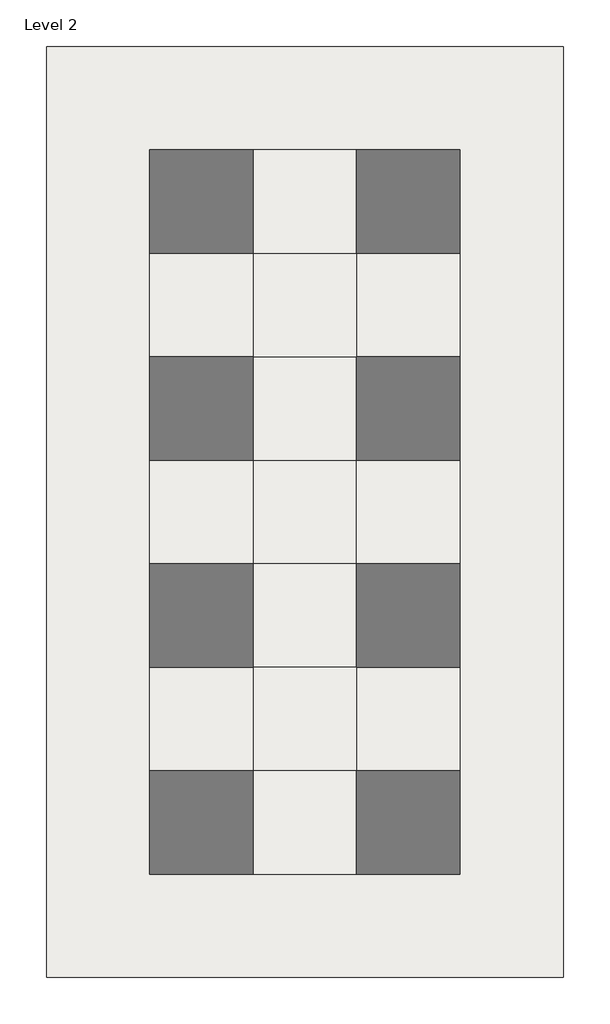
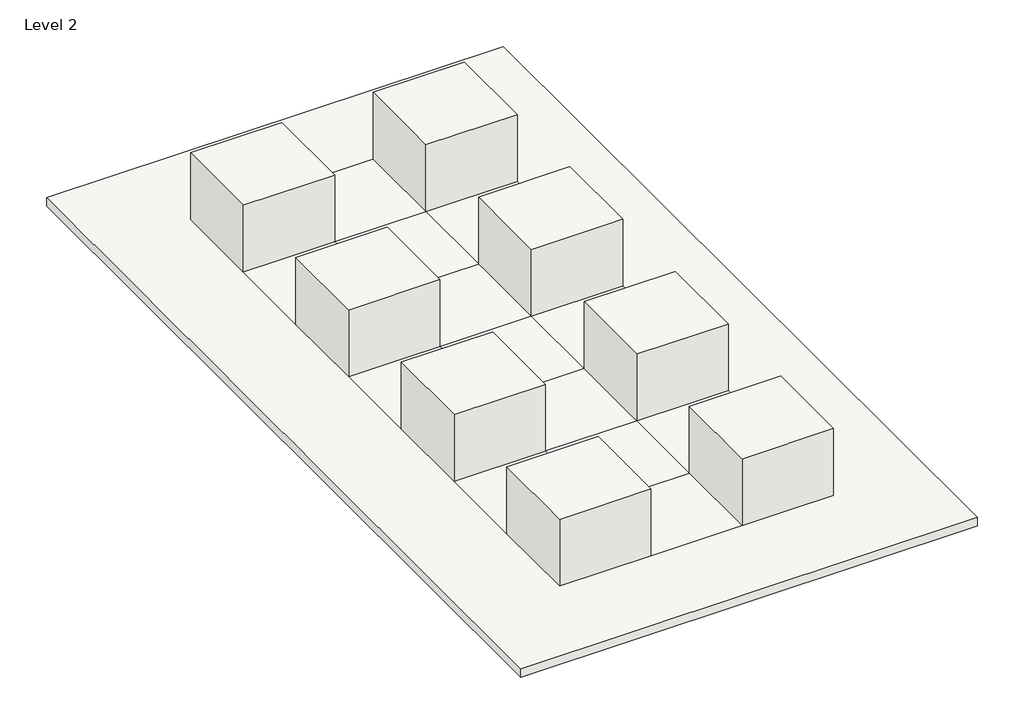
# One storey: 9 roofs.
"""IFC4 building model written with IfcOpenShell, lengths in millimetres."""

from ifc_helpers import new_model, si_unit, origin, place, context, project, spatial, faceted_brep, element, save

model = new_model("IFC4")

# Units and contexts
model_context = context("Model", 3, world=origin())
ifc_project = project(units=[si_unit("LENGTHUNIT", "METRE", prefix="MILLI")], contexts=[model_context])

# Site, building, storey
site = spatial("IfcSite", under=ifc_project)
building = spatial("IfcBuilding", under=site)
storey = spatial("IfcBuildingStorey", under=building, Name="Level 2", Elevation=8000.0)

# Roofs
placement = place(None, origin())
element("IfcRoof", 1, ObjectType="Bauder_RoofCoveringSystem_IntensiveGreenRoofSystem", at=placement, inside=storey, context=model_context, shape_type="Brep", body=[
    faceted_brep([(-674.7340554, 1676.2074539, 8000.0), (1325.2659446, 1676.2074539, 8000.0), (1325.2659446, -323.7925461, 8000.0), (-674.7340554, -323.7925461, 8000.0), (1325.2659446, 1676.2074539, 9749.8), (-674.7340554, 1676.2074539, 9749.8), (-674.7340554, -323.7925461, 9749.8), (1325.2659446, -323.7925461, 9749.8), (1325.2659446, 1676.2074539, 8200.0), (-674.7340554, 1676.2074539, 8200.0), (-674.7340554, -323.7925461, 8200.0), (1325.2659446, -323.7925461, 8200.0)], [[[0, 1, 2, 3]], [[4, 5, 6, 7]], [[5, 4, 8, 1, 0, 9]], [[6, 5, 9, 0, 3, 10]], [[7, 6, 10, 3, 2, 11]], [[4, 7, 11, 2, 1, 8]]]),
])
element("IfcRoof", 2, ObjectType="Bauder_RoofCoveringSystem_IntensiveGreenRoofSystem", at=placement, inside=storey, context=model_context, shape_type="Brep", body=[
    faceted_brep([(3325.2659446, 1676.2074539, 8000.0), (5325.2659446, 1676.2074539, 8000.0), (5325.2659446, -323.7925461, 8000.0), (3325.2659446, -323.7925461, 8000.0), (5325.2659446, 1676.2074539, 9749.8), (3325.2659446, 1676.2074539, 9749.8), (3325.2659446, -323.7925461, 9749.8), (5325.2659446, -323.7925461, 9749.8), (5325.2659446, 1676.2074539, 8200.0), (3325.2659446, 1676.2074539, 8200.0), (3325.2659446, -323.7925461, 8200.0), (5325.2659446, -323.7925461, 8200.0)], [[[0, 1, 2, 3]], [[4, 5, 6, 7]], [[5, 4, 8, 1, 0, 9]], [[6, 5, 9, 0, 3, 10]], [[7, 6, 10, 3, 2, 11]], [[4, 7, 11, 2, 1, 8]]]),
])
element("IfcRoof", 3, ObjectType="Bauder_RoofCoveringSystem_IntensiveGreenRoofSystem", at=placement, inside=storey, context=model_context, shape_type="Brep", body=[
    faceted_brep([(3325.2659446, -2323.7925461, 8000.0), (5325.2659446, -2323.7925461, 8000.0), (5325.2659446, -4323.7925461, 8000.0), (3325.2659446, -4323.7925461, 8000.0), (5325.2659446, -2323.7925461, 9749.8), (3325.2659446, -2323.7925461, 9749.8), (3325.2659446, -4323.7925461, 9749.8), (5325.2659446, -4323.7925461, 9749.8), (5325.2659446, -2323.7925461, 8200.0), (3325.2659446, -2323.7925461, 8200.0), (3325.2659446, -4323.7925461, 8200.0), (5325.2659446, -4323.7925461, 8200.0)], [[[0, 1, 2, 3]], [[4, 5, 6, 7]], [[5, 4, 8, 1, 0, 9]], [[6, 5, 9, 0, 3, 10]], [[7, 6, 10, 3, 2, 11]], [[4, 7, 11, 2, 1, 8]]]),
])
element("IfcRoof", 4, ObjectType="Bauder_RoofCoveringSystem_IntensiveGreenRoofSystem", at=placement, inside=storey, context=model_context, shape_type="Brep", body=[
    faceted_brep([(3325.2659446, -6323.7925461, 8000.0), (5325.2659446, -6323.7925461, 8000.0), (5325.2659446, -8323.7925461, 8000.0), (3325.2659446, -8323.7925461, 8000.0), (5325.2659446, -6323.7925461, 9749.8), (3325.2659446, -6323.7925461, 9749.8), (3325.2659446, -8323.7925461, 9749.8), (5325.2659446, -8323.7925461, 9749.8), (5325.2659446, -6323.7925461, 8200.0), (3325.2659446, -6323.7925461, 8200.0), (3325.2659446, -8323.7925461, 8200.0), (5325.2659446, -8323.7925461, 8200.0)], [[[0, 1, 2, 3]], [[4, 5, 6, 7]], [[5, 4, 8, 1, 0, 9]], [[6, 5, 9, 0, 3, 10]], [[7, 6, 10, 3, 2, 11]], [[4, 7, 11, 2, 1, 8]]]),
])
element("IfcRoof", 5, ObjectType="Bauder_RoofCoveringSystem_IntensiveGreenRoofSystem", at=placement, inside=storey, context=model_context, shape_type="Brep", body=[
    faceted_brep([(3325.2659446, -10323.7925461, 8000.0), (5325.2659446, -10323.7925461, 8000.0), (5325.2659446, -12323.7925461, 8000.0), (3325.2659446, -12323.7925461, 8000.0), (5325.2659446, -10323.7925461, 9749.8), (3325.2659446, -10323.7925461, 9749.8), (3325.2659446, -12323.7925461, 9749.8), (5325.2659446, -12323.7925461, 9749.8), (5325.2659446, -10323.7925461, 8200.0), (3325.2659446, -10323.7925461, 8200.0), (3325.2659446, -12323.7925461, 8200.0), (5325.2659446, -12323.7925461, 8200.0)], [[[0, 1, 2, 3]], [[4, 5, 6, 7]], [[5, 4, 8, 1, 0, 9]], [[6, 5, 9, 0, 3, 10]], [[7, 6, 10, 3, 2, 11]], [[4, 7, 11, 2, 1, 8]]]),
])
element("IfcRoof", 6, ObjectType="Bauder_RoofCoveringSystem_IntensiveGreenRoofSystem", at=placement, inside=storey, context=model_context, shape_type="Brep", body=[
    faceted_brep([(-674.7340554, -10323.7925461, 8000.0), (1325.2659446, -10323.7925461, 8000.0), (1325.2659446, -12323.7925461, 8000.0), (-674.7340554, -12323.7925461, 8000.0), (1325.2659446, -10323.7925461, 9749.8), (-674.7340554, -10323.7925461, 9749.8), (-674.7340554, -12323.7925461, 9749.8), (1325.2659446, -12323.7925461, 9749.8), (1325.2659446, -10323.7925461, 8200.0), (-674.7340554, -10323.7925461, 8200.0), (-674.7340554, -12323.7925461, 8200.0), (1325.2659446, -12323.7925461, 8200.0)], [[[0, 1, 2, 3]], [[4, 5, 6, 7]], [[5, 4, 8, 1, 0, 9]], [[6, 5, 9, 0, 3, 10]], [[7, 6, 10, 3, 2, 11]], [[4, 7, 11, 2, 1, 8]]]),
])
element("IfcRoof", 7, ObjectType="Bauder_RoofCoveringSystem_IntensiveGreenRoofSystem", at=placement, inside=storey, context=model_context, shape_type="Brep", body=[
    faceted_brep([(-674.7340554, -6323.7925461, 8000.0), (1325.2659446, -6323.7925461, 8000.0), (1325.2659446, -8323.7925461, 8000.0), (-674.7340554, -8323.7925461, 8000.0), (1325.2659446, -6323.7925461, 9749.8), (-674.7340554, -6323.7925461, 9749.8), (-674.7340554, -8323.7925461, 9749.8), (1325.2659446, -8323.7925461, 9749.8), (1325.2659446, -6323.7925461, 8200.0), (-674.7340554, -6323.7925461, 8200.0), (-674.7340554, -8323.7925461, 8200.0), (1325.2659446, -8323.7925461, 8200.0)], [[[0, 1, 2, 3]], [[4, 5, 6, 7]], [[5, 4, 8, 1, 0, 9]], [[6, 5, 9, 0, 3, 10]], [[7, 6, 10, 3, 2, 11]], [[4, 7, 11, 2, 1, 8]]]),
])
element("IfcRoof", 8, ObjectType="Bauder_RoofCoveringSystem_IntensiveGreenRoofSystem", at=placement, inside=storey, context=model_context, shape_type="Brep", body=[
    faceted_brep([(-674.7340554, -2323.7925461, 8000.0), (1325.2659446, -2323.7925461, 8000.0), (1325.2659446, -4323.7925461, 8000.0), (-674.7340554, -4323.7925461, 8000.0), (1325.2659446, -2323.7925461, 9749.8), (-674.7340554, -2323.7925461, 9749.8), (-674.7340554, -4323.7925461, 9749.8), (1325.2659446, -4323.7925461, 9749.8), (1325.2659446, -2323.7925461, 8200.0), (-674.7340554, -2323.7925461, 8200.0), (-674.7340554, -4323.7925461, 8200.0), (1325.2659446, -4323.7925461, 8200.0)], [[[0, 1, 2, 3]], [[4, 5, 6, 7]], [[5, 4, 8, 1, 0, 9]], [[6, 5, 9, 0, 3, 10]], [[7, 6, 10, 3, 2, 11]], [[4, 7, 11, 2, 1, 8]]]),
])
element("IfcRoof", 9, ObjectType="Roof_Concrete-200mm", at=placement, inside=storey, context=model_context, shape_type="Brep", body=[
    faceted_brep([(-2674.7340554, -14323.7925461, 8200.0), (-2674.7340554, -14323.7925461, 8000.0), (7325.2659446, -14323.7925461, 8000.0), (7325.2659446, -14323.7925461, 8200.0), (-2674.7340554, 3676.2074539, 8200.0), (-2674.7340554, 3676.2074539, 8000.0), (7325.2659446, 3676.2074539, 8200.0), (7325.2659446, 3676.2074539, 8000.0), (3325.2659446, 1676.2074539, 8200.0), (1325.2659446, 1676.2074539, 8200.0), (1325.2659446, -323.7925461, 8200.0), (3325.2659446, -323.7925461, 8200.0), (1325.2659446, 1676.2074539, 8000.0), (3325.2659446, 1676.2074539, 8000.0), (3325.2659446, -323.7925461, 8000.0), (1325.2659446, -323.7925461, 8000.0), (1325.2659446, -2323.7925461, 8200.0), (-674.7340554, -323.7925461, 8200.0), (-674.7340554, -2323.7925461, 8200.0), (3325.2659446, -2323.7925461, 8200.0), (5325.2659446, -2323.7925461, 8200.0), (5325.2659446, -323.7925461, 8200.0), (-674.7340554, -2323.7925461, 8000.0), (-674.7340554, -323.7925461, 8000.0), (1325.2659446, -2323.7925461, 8000.0), (3325.2659446, -2323.7925461, 8000.0), (5325.2659446, -323.7925461, 8000.0), (5325.2659446, -2323.7925461, 8000.0), (1325.2659446, -4323.7925461, 8200.0), (3325.2659446, -4323.7925461, 8200.0), (3325.2659446, -4323.7925461, 8000.0), (1325.2659446, -4323.7925461, 8000.0), (1325.2659446, -6323.7925461, 8200.0), (-674.7340554, -4323.7925461, 8200.0), (-674.7340554, -6323.7925461, 8200.0), (5325.2659446, -6323.7925461, 8200.0), (5325.2659446, -4323.7925461, 8200.0), (3325.2659446, -6323.7925461, 8200.0), (-674.7340554, -6323.7925461, 8000.0), (-674.7340554, -4323.7925461, 8000.0), (1325.2659446, -6323.7925461, 8000.0), (3325.2659446, -6323.7925461, 8000.0), (5325.2659446, -4323.7925461, 8000.0), (5325.2659446, -6323.7925461, 8000.0), (1325.2659446, -12323.7925461, 8200.0), (3325.2659446, -12323.7925461, 8200.0), (3325.2659446, -10323.7925461, 8200.0), (1325.2659446, -10323.7925461, 8200.0), (3325.2659446, -12323.7925461, 8000.0), (1325.2659446, -12323.7925461, 8000.0), (1325.2659446, -10323.7925461, 8000.0), (3325.2659446, -10323.7925461, 8000.0), (1325.2659446, -8323.7925461, 8200.0), (-674.7340554, -8323.7925461, 8200.0), (-674.7340554, -10323.7925461, 8200.0), (3325.2659446, -8323.7925461, 8200.0), (5325.2659446, -10323.7925461, 8200.0), (5325.2659446, -8323.7925461, 8200.0), (-674.7340554, -10323.7925461, 8000.0), (-674.7340554, -8323.7925461, 8000.0), (1325.2659446, -8323.7925461, 8000.0), (3325.2659446, -8323.7925461, 8000.0), (5325.2659446, -8323.7925461, 8000.0), (5325.2659446, -10323.7925461, 8000.0), (-674.7340554, 1676.2074539, 8000.0), (-674.7340554, 1676.2074539, 8200.0), (5325.2659446, 1676.2074539, 8200.0), (5325.2659446, 1676.2074539, 8000.0), (5325.2659446, -12323.7925461, 8000.0), (5325.2659446, -12323.7925461, 8200.0), (-674.7340554, -12323.7925461, 8000.0), (-674.7340554, -12323.7925461, 8200.0)], [[[0, 1, 2, 3]], [[1, 0, 4, 5]], [[6, 7, 5, 4]], [[3, 2, 7, 6]], [[8, 9, 10, 11]], [[12, 13, 14, 15]], [[16, 10, 17, 18]], [[11, 10, 16, 19]], [[20, 21, 11, 19]], [[22, 23, 15, 24]], [[15, 14, 25, 24]], [[25, 14, 26, 27]], [[19, 16, 28, 29]], [[24, 25, 30, 31]], [[32, 28, 33, 34]], [[35, 36, 29, 37]], [[38, 39, 31, 40]], [[41, 30, 42, 43]], [[44, 45, 46, 47]], [[48, 49, 50, 51]], [[47, 52, 53, 54]], [[47, 46, 55, 52]], [[56, 57, 55, 46]], [[58, 59, 60, 50]], [[51, 50, 60, 61]], [[51, 61, 62, 63]], [[52, 55, 37, 32]], [[29, 28, 32, 37]], [[61, 60, 40, 41]], [[31, 30, 41, 40]], [[9, 12, 15, 10]], [[10, 15, 23, 17]], [[17, 23, 64, 65]], [[12, 9, 65, 64]], [[66, 67, 26, 21]], [[21, 26, 14, 11]], [[11, 14, 13, 8]], [[67, 66, 8, 13]], [[20, 27, 42, 36]], [[36, 42, 30, 29]], [[29, 30, 25, 19]], [[27, 20, 19, 25]], [[16, 24, 31, 28]], [[28, 31, 39, 33]], [[33, 39, 22, 18]], [[24, 16, 18, 22]], [[32, 40, 60, 52]], [[52, 60, 59, 53]], [[53, 59, 38, 34]], [[40, 32, 34, 38]], [[35, 43, 62, 57]], [[57, 62, 61, 55]], [[55, 61, 41, 37]], [[43, 35, 37, 41]], [[56, 63, 68, 69]], [[69, 68, 48, 45]], [[45, 48, 51, 46]], [[63, 56, 46, 51]], [[47, 50, 49, 44]], [[44, 49, 70, 71]], [[71, 70, 58, 54]], [[50, 47, 54, 58]], [[4, 0, 3, 6], [9, 8, 66, 21, 20, 36, 35, 57, 56, 69, 45, 44, 71, 54, 53, 34, 33, 18, 17, 65]], [[7, 2, 1, 5], [13, 12, 64, 23, 22, 39, 38, 59, 58, 70, 49, 48, 68, 63, 62, 43, 42, 27, 26, 67]]]),
])

save(model, "model.ifc")

# Revit data of these elements
# Type "Bauder_RoofCoveringSystem_IntensiveGreenRoofSystem"
#   Keynote = "Q37"
#   Type IFC Predefined Type = "FLAT_ROOF"
#   Export Type to IFC As = "IfcRoofType"
#   Model = "Bauder Intensive Landscaping and Substrate - Intensive Green Roof System"
#   Manufacturer = "Bauder Ltd"
#   Type Comments = "Intensive Green Roof System"
#   URL = "http://www.bauder.co.uk/"
#   Description = "Bauder Intensive GreenRoof system incorporating Intensive Landscaping with Intensive Substrate, Filter Fleece, Mineral Drain, DSE60 Polyethylene Drainage and Protection Layer, FSM 1100 protection mat and PE Foil Polyethylene Separation-Slip Layer"
#   Assembly Code = "B3010"
#   NBSDescription = "Intensive green roof system"
#   NBSReference = "45-40-47/110"
#   BIMObjectName = "Bauder_RoofCoveringSystem_IntensiveGreenRoofSystem"
#   AccessibilityPerformance = "n/a"
#   CodePerformance = "n/a"
#   Color = "n/a"
#   Constituents = "n/a"
#   DurationUnit = "Year"
#   ExpectedLife = "n/a"
#   Features = "This BIM Object must be supported by a project specific specification from Bauder, incorporating system build-up, detail design and performance calculations if a full Bauder system guarantee is required. Please contact your local Bauder Representative or technical@bauder.co.uk"
#   Finish = "n/a"
#   Grade = "n/a"
#   Material = "n/a"
#   ModelReference = "Bauder Intensive Landscaping and Substrate - Intensive Green Roof System"
#   Name = "RoofCoveringSystem_Bauder_IntensiveGreenRoofSystem"
#   ReplacementCost = "n/a"
#   Shape = "n/a"
#   Size = "n/a"
#   SustainabilityPerformance = "Bauder Germany ISO14001: Certificate No.: 70499/03-15 e, Bauder UK ISO14001:Certificate No. 19ACM6595R, EN1271, BREEAM Credits Available"
#   WarrantyDescription = "Guarantee options could include ‘Product’, ‘Product and Workmanship’ and ‘Product, Workmanship and Design’ Guarantees. All guarantees available for this system are subject to the works being carried out in accordance with the Bauder specification and being installed by a Bauder Approved installer. For full details and further information regarding guarantees and alternative systems please contact your local Bauder Representative or technical@bauder.co.uk"
#   WarrantyDurationLabor = "n/a"
#   WarrantyDurationParts = "n/a\r\nn/a"
#   WarrantyDurationUnit = "Year"
#   WarrantyGuarantorLabor = "n/a"
#   WarrantyGuarantorParts = "technical@bauder.co.uk"
#   Certification = "n/a"
#   EdgeRestraints = "Perforated edge trim where required, refer to Bauder Project Specific Specification"
#   MoistureControlDrainageAncillaries = "n/a"
#   MoistureControlDrainageLayer = "Bauder DSE60 60 mm Polyethylene Drainage and Protection Layer with Bauder Mineral Drain Single size stone aggregate infill"
#   MoistureControlFilterMembrane = "Bauder Filter Fleece 1 mm Polypropylene Filter Fleece"
#   MoistureControlMoistureRetentionMat = "n/a"
#   PlantingSystemsAntierosionMat = "Jute Net where exposed, refer to Bauder Project Specific Specification"
#   PlantingSystemsPlantingMedium = "Bauder Intensive Substrate Recycled crushed brick, expanded clay shale and composted pine bark"
#   PlantingSystemsVegetation = "Bauder Intensive Landscaping"
#   PlantingSystemsVegetationBarrier = "20-40 mm Rounded-Washed Stones, refer to Bauder Project Specific Specification"
#   ProjectSpecificationAndDesign = "This BIM Object must be supported by a project specific specification from Bauder, incorporating system build-up, detail design and performance calculations if a full Bauder system warranty is required. Please contact your local Bauder Representative or technical@bauder.co.uk"
#   ProtectionProtectionLayer = "BauderGREEN FSM 1100 Protection Mat"
#   ProtectionRootBarrier = "As per project specific Bauder Specification"
#   ProtectionSeparationLayer = "2 layers of Bauder PE Foil 0.2 mm Polyethylene Separation-Slip Layer"
#   SystemManufacturer = "Bauder Ltd"
#   WarrantyConsiderations = "All guarantees available for this system are subject to the works being carried out in accordance with the Bauder specification and being installed by a Bauder Approved installer. For full details and further information regarding guarantees and alternative systems please contact your local Bauder Representative or technical@bauder.co.uk"
#   Update = "1900-12-31T23:59:59"
#   Documentation = "https://www.bauder.co.uk/technical-centre/technical-literature/system-brochures"
#   DocumentReference = "http://www.bauder.co.uk/"
#   IfcExportAs = "IfcRoofType"
#   IfcExportType = "FLAT_ROOF"
#   MethodOfMesurement = "n/a"
#   Process = "Replacement at service life intervals"
#   FireRating = "n/a"
#   _Author = "AM"
#   _AuthorizedBy = "bimstore"
#   _CreatedBy = "technical@bauder.co.uk"
#   _DistributedBy = "www.bimstore.co"
#   AssetType = "Fixed"
#   ClassificationName = "Uniclass2015"
#   ClassificationValue = "Ss_45_40_47_40"
#   CreatedBy = "technical@bauder.co.uk"
#   CreatedOn = "2023-02-10 T00:00:00"
#   DocumentationCertificates = "n/a"
#   DocumentationInstallationGuide = "https://www.bauder.co.uk/technical-centre"
#   DocumentationLiterature = "https://www.bauder.co.uk/technical-centre"
#   DocumentationMaintenance = "https://www.bauder.co.uk/technical-centre/maintenance-advice"
#   DocumentationTechnical = "https://www.bauder.co.uk/green-roofs/intensive-green-roofs"
#   ManufacturerName = "Bauder Ltd"
#   ModelNumber = "0910_INT-InS-FF-D6-F11-PE"
#   ProductionYear = "2023"
#   ReferencedStandard = "n/a"
#   SpareParts = "n/a"
#   TypeName = "Intensive Green Roof System"
#   NBSNote = "n/a"
#   NBSObjectName = "Bauder - Intensive green roof system"
#   NBSOfficeMasterTag = "n/a"
#   Ballast = "n/a"
#   CarrierMembraneFixing = "n/a"
#   CarrierMembraneType = "n/a"
#   FillToPerimeterUpstands = "n/a"
#   FilterLayer = "n/a"
#   InsulationFixing = "n/a"
#   InsulationType = "n/a"
#   LiquidAppliedWaterproofCoatingReinforcement = "n/a"
#   LiquidAppliedWaterproofCoatingSurfaceTreatment = "n/a"
#   LiquidAppliedWaterproofCoatingType = "n/a"
#   PreparationExistingSubstrates = "n/a"
#   PreparationHorizontalWork = "n/a"
#   PreparationSkirtingsAndVerticalWork = "n/a"
#   ProtectionLayer = "n/a"
#   SystemAccessories = "n/a"
#   WaterproofCoveringFirstLayerAttachment = "n/a"
#   WaterproofCoveringFirstLayerType = "n/a"
#   WaterproofCoveringIntermediateLayerAttachment = "n/a"
#   WaterproofCoveringIntermediateLayerType = "n/a"
#   WaterproofCoveringTopLayerAttachment = "n/a"
#   InsulationAttachment = "n/a"
#   IsolatingLayer = "n/a"
#   CarrierMembraneAttachment = "n/a"
#   LiquidAppliedWaterproofCoatingWearingCourse = "n/a"
#   VapourControlLayer = "n/a"
#   VapourControlLayerAttachment_Bauder = "n/a"
#   WaterproofCoveringJoints = "n/a"
#   WaterproofCoveringType = "n/a"
#   SeparatingLayer = "n/a"
#   WaterproofCoveringAccessories = "Yes"
#   WaterproofCoveringAttachment = "n/a"
#   UpperProtectionLayer = "n/a"
#   LowerProtectionLayer = "n/a"
#   WaterproofCoveringTopLayerType = "n/a"
#   DetailWorkAncillaryItems = "Detail as per project specific Bauder Specification"
#   DetailWorkCoverStrips = "Detail as per project specific Bauder Specification"
#   DetailWorkFlashings = "Detail as per project specific Bauder Specification"
#   DetailWorkSkirtingsAndUpstands = "Detail as per project specific Bauder Specification"
#   DetailWorkWeltedDrips = "Detail as per project specific Bauder Specification"
#   OverlayFixing = "n/a"
#   OverlayType = "n/a"
#   SurfaceProtection = "n/a"
#   VapourControlLayerAttachment = "n/a"
#   VapourControlLayerType = "n/a"
#   Cost = 0
#   NominalHeight = 0 mm
#   NominalLength = 0 mm
#   TotalArea = 0 m²
#   NominalDepth = 0 mm
#   IsExternal = yes
#   _BimSpecGuid = 0
#   _BSBibleVersion = 16
#   _CurrentRevision = 4
#   Layers, outside or top first: 700 mm "Bauder_Landscaping_Intensive" (function 5); 800 mm "Bauder_IntensiveSubstrate_BauderGREEN-SUB-IM-UK" (function 2); 1 mm "Bauder_FilterFleece_BauderGREEN-FV-125-100" (function 2); 40 mm "Bauder_DrainageBoard_BauderGREEN-DSE-40" (function 3); 8 mm "Bauder_ProtectionMat_BauderGREEN-FSM1100" (function 3); 200 mm "Concrete" (function 1); 0.8 mm "Bauder_SeparationAndSlipLayer_BauderGREEN-PE-02" (function 3)
# Type "Roof_Concrete-200mm"
#   Layers, outside or top first: 200 mm "Concrete" (function 1)
# Elements 1, 2, 3, 4, 5, 6, 7, 8 (IfcRoof, "Bauder_RoofCoveringSystem_IntensiveGreenRoofSystem")
#   built-in parameter 1001705 = 31.9875 (stored number, unit not read)
#   built-in parameter 1001710 = 33615
#   Phase Created = New Construction
#   Materials on its faces: "Bauder_SeparationAndSlipLayer_BauderGREEN-PE-02", "Bauder_Landscaping_Intensive"
# Element 9 (IfcRoof, "Roof_Concrete-200mm")
#   built-in parameter 1001710 = 33615
#   Phase Created = New Construction
#   Materials on its faces: "Concrete"
# Materials
#   "Bauder_Landscaping_Intensive": class "Unassigned", colour RGB 62 68 37, transparency 0, Mtrl_Author = "AM", Mtrl_AuthorizedBy = "bimstore", Mtrl_DistributedBy = "www.bimstore.co", Mtrl_AccessibilityPerformance = "n/a", Mtrl_AssetIdentifier = "Please record on commissioning", Mtrl_AssetType = "Fixed", Mtrl_BarCode = "Please record on commissioning", Mtrl_ClassificationName = "Uniclass2015", Mtrl_ClassificationValue = "n/a", Mtrl_CodePerformance = "n/a", Mtrl_Color = "n/a", Mtrl_Constituents = "n/a", Mtrl_CreatedBy = "technical@bauder.co.uk", Mtrl_CreatedOn = "2023-02-10 T00:00:00", Mtrl_DocumentationCertificates = "https://www.bimstore.co/products/intensive-green-roof-system/document/product-certificates", Mtrl_DocumentationInstallationGuide = "https://www.bimstore.co/products/intensive-green-roof-system/document/installation-guide", Mtrl_DocumentationLiterature = "https://www.bimstore.co/products/intensive-green-roof-system/document/product-literature", Mtrl_DocumentationMaintenance = "https://www.bimstore.co/products/intensive-green-roof-system/document/maintenance-information", Mtrl_DocumentationTechnical = "https://www.bimstore.co/products/intensive-green-roof-system/document/technical-data-sheet", Mtrl_DurationUnit = "Year", Mtrl_Features = "n/a", Mtrl_Finish = "n/a", Mtrl_Grade = "n/a", Mtrl_InstallationDate = "Please record on commissioning", Mtrl_ManufacturerName = "Bauder Ltd", Mtrl_Material = "n/a", Mtrl_ModelNumber = "Intensive", Mtrl_ModelReference = "Landscaping", Mtrl_ProductionYear = "2023", Mtrl_ReferencedStandard = "n/a", Mtrl_Shape = "n/a", Mtrl_Size = "n/a", Mtrl_SpareParts = "n/a", Mtrl_TypeName = "Intensive", Mtrl_WarrantyDescription = "n/a", Mtrl_WarrantyDurationUnit = "Year", Mtrl_WarrantyGuarantorLabor = "n/a", Mtrl_WarrantyGuarantorParts = "technical@bauder.co.uk", Mtrl_WarrantyStartDate = "Please record on commissioning", Mtrl_IfcExportAs = "IfcRoofType", Mtrl_IfcExportType = "FLAT_ROOF", Mtrl_BIMObjectName = "Bauder_Landscaping_Intensive", Mtrl_NBSDescription = "n/a", Mtrl_NBSNote = "n/a", Mtrl_NBSObjectName = "n/a", Mtrl_NBSOfficeMasterTag = "n/a", Mtrl_NBSReference = "Q37", Mtrl_Ballast = "n/a", Mtrl_CarrierMembraneAttachment = "n/a", Mtrl_CarrierMembraneFixing = "n/a", Mtrl_CarrierMembraneType = "n/a", Mtrl_Certification = "Comply with GRO Green Roof Code of Practice and FLL Standards", Mtrl_DetailWorkAncillaryItems = "Detail as per project specific Bauder Specification", Mtrl_DetailWorkCoverStrips = "Detail as per project specific Bauder Specification", Mtrl_DetailWorkFlashings = "Detail as per project specific Bauder Specification", Mtrl_DetailWorkSkirtingsAndUpstands = "Detail as per project specific Bauder Specification", Mtrl_DetailWorkWeltedDrips = "Detail as per project specific Bauder Specification", Mtrl_EdgeRestraints = "Detail as per project specific Bauder Specification", Mtrl_FillToPerimeterUpstands = "n/a", Mtrl_FilterLayer = "n/a", Mtrl_InsulationAttachment = "As per project specific Bauder Specification", Mtrl_InsulationFixing = "As per project specific Bauder Specification", Mtrl_InsulationType = "As per project specific Bauder Specification", Mtrl_IsolatingLayer = "n/a", Mtrl_LiquidAppliedWaterproofCoatingReinforcement = "n/a", Mtrl_LiquidAppliedWaterproofCoatingSurfaceTreatment = "As per project specific Bauder Specification", Mtrl_LiquidAppliedWaterproofCoatingType = "As per project specific Bauder Specification", Mtrl_LiquidAppliedWaterproofCoatingWearingCourse = "As per project specific Bauder Specification", Mtrl_LowerProtectionLayer = "n/a", Mtrl_MoistureControlDrainageAncillaries = "n/a", Mtrl_MoistureControlDrainageLayer = "n/a", Mtrl_MoistureControlFilterMembrane = "n/a", Mtrl_MoistureControlMoistureRetentionMat = "n/a", Mtrl_OverlayFixing = "n/a", Mtrl_OverlayType = "n/a", Mtrl_PlantingSystemsAntierosionMat = "n/a", Mtrl_PlantingSystemsPlantingMedium = "As per project specific Bauder Specification", Mtrl_PlantingSystemsVegetation = "As per project specific Bauder Specification", Mtrl_PlantingSystemsVegetationBarrier = "As per project specific Bauder Specification", Mtrl_PreparationExistingSubstrates = "n/a", Mtrl_PreparationHorizontalWork = "n/a", Mtrl_PreparationSkirtingsAndVerticalWork = "n/a", Mtrl_ProjectSpecificationAndDesign = "This BIM Object must be supported by a project specific specification from Bauder, incorporating system build-up, detail design and performance calculations if a full Bauder system warranty is required. Please contact your local Bauder Representative or technical@bauder.co.uk", Mtrl_ProtectionLayer = "n/a", Mtrl_ProtectionProtectionLayer = "n/a", Mtrl_ProtectionRootBarrier = "As per project specific Bauder Specification", Mtrl_ProtectionSeparationLayer = "n/a", Mtrl_SeparatingLayer = "n/a", Mtrl_SurfaceProtection = "n/a", Mtrl_SystemAccessories = "n/a", Mtrl_SystemManufacturer = "Bauder Ltd", Mtrl_Update = "1900-12-31 T23:59:59", Mtrl_UpperProtectionLayer = "n/a", Mtrl_VapourControlLayerAttachment = "As per project specific Bauder Specification", Mtrl_VapourControlLayerAttachment_Bauder = "As per project specific Bauder Specification", Mtrl_VapourControlLayerType = "As per project specific Bauder Specification", Mtrl_WarrantyConsiderations = "All guarantees available for this system are subject to the works being carried out in accordance with the Bauder specification and being installed by a Bauder Approved installer. For full details and further information regarding guarantees and alternative systems please contact your local Bauder Representative or technical@bauder.co.uk", Mtrl_WaterproofCoveringAccessories = "As per project specific Bauder Specification", Mtrl_WaterproofCoveringAttachment = "As per project specific Bauder Specification", Mtrl_WaterproofCoveringFirstLayerAttachment = "As per project specific Bauder Specification", Mtrl_WaterproofCoveringFirstLayerType = "As per project specific Bauder Specification", Mtrl_WaterproofCoveringIntermediateLayerAttachment = "As per project specific Bauder Specification", Mtrl_WaterproofCoveringIntermediateLayerType = "As per project specific Bauder Specification", Mtrl_WaterproofCoveringJoints = "As per project specific Bauder Specification", Mtrl_WaterproofCoveringTopLayerAttachment = "As per project specific Bauder Specification", Mtrl_WaterproofCoveringTopLayerType = "As per project specific Bauder Specification", Mtrl_WaterproofCoveringType = "As per project specific Bauder Specification", Cost = 0, Mtrl_ReplacementCost = 0, Mtrl_NominalDepth = 0 mm, Mtrl_NominalHeight = 0 mm, Mtrl_NominalLength = 0 mm, Mtrl_BimSpecGuid = 0, Mtrl_BSBibleVersion = 17, Mtrl_CurrentRevision = 2, Mtrl_ExpectedLife = 0, Mtrl_SerialNumber = 0, Mtrl_WarrantyDurationLabor = 0, Mtrl_WarrantyDurationParts = 0
#   "Bauder_IntensiveSubstrate_BauderGREEN-SUB-IM-UK": class "Unassigned", colour RGB 255 255 255, transparency 0, Mtrl_Author = "AM", Mtrl_AuthorizedBy = "bimstore", Mtrl_DistributedBy = "www.bimstore.co", Mtrl_AccessibilityPerformance = "n/a", Mtrl_AssetIdentifier = "Please record on commissioning", Mtrl_AssetType = "Fixed", Mtrl_BarCode = "Please record on commissioning", Mtrl_ClassificationName = "Uniclass2015", Mtrl_ClassificationValue = "n/a", Mtrl_CodePerformance = "n/a", Mtrl_Color = "n/a", Mtrl_Constituents = "n/a", Mtrl_CreatedBy = "technical@bauder.co.uk", Mtrl_CreatedOn = "2023-02-10 T00:00:00", Mtrl_DocumentationCertificates = "https://www.bimstore.co/products/intensive-green-roof-system/document/product-certificates", Mtrl_DocumentationInstallationGuide = "https://www.bimstore.co/products/intensive-green-roof-system/document/installation-guide", Mtrl_DocumentationLiterature = "https://www.bimstore.co/products/intensive-green-roof-system/document/product-literature", Mtrl_DocumentationMaintenance = "https://www.bimstore.co/products/intensive-green-roof-system/document/maintenance-information", Mtrl_DocumentationTechnical = "https://www.bimstore.co/products/intensive-green-roof-system/document/technical-data-sheet", Mtrl_DurationUnit = "Year", Mtrl_Features = "n/a", Mtrl_Finish = "n/a", Mtrl_Grade = "n/a", Mtrl_InstallationDate = "Please record on commissioning", Mtrl_ManufacturerName = "Bauder Ltd", Mtrl_Material = "Expanded Clay Aggregate", Mtrl_ModelNumber = "BauderGREEN-SUB-IM-UK", Mtrl_ModelReference = "Intensive Substrate", Mtrl_ProductionYear = "2023", Mtrl_ReferencedStandard = "n/a", Mtrl_Shape = "n/a", Mtrl_Size = "n/a", Mtrl_SpareParts = "n/a", Mtrl_TypeName = "BauderGREEN-SUB-IM-UK", Mtrl_WarrantyDescription = "As part of Bauder system guarantee, per specification", Mtrl_WarrantyDurationUnit = "Year", Mtrl_WarrantyGuarantorLabor = "n/a", Mtrl_WarrantyGuarantorParts = "technical@bauder.co.uk", Mtrl_WarrantyStartDate = "Please record on commissioning", Mtrl_IfcExportAs = "IfcRoofType", Mtrl_IfcExportType = "FLAT_ROOF", Mtrl_BIMObjectName = "Bauder_IntensiveSubstrate_BauderGREEN-SUB-IM-UK", Mtrl_NBSDescription = "n/a", Mtrl_NBSNote = "n/a", Mtrl_NBSObjectName = "n/a", Mtrl_NBSOfficeMasterTag = "n/a", Mtrl_NBSReference = "Q37", Mtrl_Ballast = "n/a", Mtrl_CarrierMembraneAttachment = "n/a", Mtrl_CarrierMembraneFixing = "n/a", Mtrl_CarrierMembraneType = "n/a", Mtrl_Certification = "Comply with GRO Green Roof Code of Practice and FLL Standards", Mtrl_DetailWorkAncillaryItems = "Detail as per project specific Bauder Specification", Mtrl_DetailWorkCoverStrips = "Detail as per project specific Bauder Specification", Mtrl_DetailWorkFlashings = "Detail as per project specific Bauder Specification", Mtrl_DetailWorkSkirtingsAndUpstands = "Detail as per project specific Bauder Specification", Mtrl_DetailWorkWeltedDrips = "Detail as per project specific Bauder Specification", Mtrl_EdgeRestraints = "Detail as per project specific Bauder Specification", Mtrl_FillToPerimeterUpstands = "n/a", Mtrl_FilterLayer = "n/a", Mtrl_InsulationAttachment = "As per project specific Bauder Specification", Mtrl_InsulationFixing = "As per project specific Bauder Specification", Mtrl_InsulationType = "As per project specific Bauder Specification", Mtrl_IsolatingLayer = "n/a", Mtrl_LiquidAppliedWaterproofCoatingReinforcement = "As per project specific Bauder Specification", Mtrl_LiquidAppliedWaterproofCoatingSurfaceTreatment = "As per project specific Bauder Specification", Mtrl_LiquidAppliedWaterproofCoatingType = "As per project specific Bauder Specification", Mtrl_LiquidAppliedWaterproofCoatingWearingCourse = "As per project specific Bauder Specification", Mtrl_LowerProtectionLayer = "n/a", Mtrl_MoistureControlDrainageAncillaries = "n/a", Mtrl_MoistureControlDrainageLayer = "n/a", Mtrl_MoistureControlFilterMembrane = "n/a", Mtrl_MoistureControlMoistureRetentionMat = "n/a", Mtrl_OverlayFixing = "n/a", Mtrl_OverlayType = "n/a", Mtrl_PlantingSystemsAntierosionMat = "n/a", Mtrl_PlantingSystemsPlantingMedium = "As per project specific Bauder Specification", Mtrl_PlantingSystemsVegetation = "As per project specific Bauder Specification", Mtrl_PlantingSystemsVegetationBarrier = "As per project specific Bauder Specification", Mtrl_PreparationExistingSubstrates = "n/a", Mtrl_PreparationHorizontalWork = "n/a", Mtrl_PreparationSkirtingsAndVerticalWork = "n/a", Mtrl_ProjectSpecificationAndDesign = "This BIM Object must be supported by a project specific specification from Bauder, incorporating system build-up, detail design and performance calculations if a full Bauder system warranty is required. Please contact your local Bauder Representative or technical@bauder.co.uk", Mtrl_ProtectionLayer = "n/a", Mtrl_ProtectionProtectionLayer = "n/a", Mtrl_ProtectionRootBarrier = "As per project specific Bauder Specification", Mtrl_ProtectionSeparationLayer = "n/a", Mtrl_SeparatingLayer = "n/a", Mtrl_SurfaceProtection = "n/a", Mtrl_SystemAccessories = "n/a", Mtrl_SystemManufacturer = "Bauder Ltd", Mtrl_Update = "1900-12-31 T23:59:59", Mtrl_UpperProtectionLayer = "n/a", Mtrl_VapourControlLayerAttachment = "As per project specific Bauder Specification", Mtrl_VapourControlLayerAttachment_Bauder = "As per project specific Bauder Specification", Mtrl_VapourControlLayerType = "As per project specific Bauder Specification", Mtrl_WarrantyConsiderations = "All guarantees available for this system are subject to the works being carried out in accordance with the Bauder specification and being installed by a Bauder Approved installer. For full details and further information regarding guarantees and alternative systems please contact your local Bauder Representative or technical@bauder.co.uk", Mtrl_WaterproofCoveringAccessories = "As per project specific Bauder Specification", Mtrl_WaterproofCoveringAttachment = "As per project specific Bauder Specification", Mtrl_WaterproofCoveringFirstLayerAttachment = "As per project specific Bauder Specification", Mtrl_WaterproofCoveringFirstLayerType = "As per project specific Bauder Specification", Mtrl_WaterproofCoveringIntermediateLayerAttachment = "As per project specific Bauder Specification", Mtrl_WaterproofCoveringIntermediateLayerType = "As per project specific Bauder Specification", Mtrl_WaterproofCoveringJoints = "As per project specific Bauder Specification", Mtrl_WaterproofCoveringTopLayerAttachment = "As per project specific Bauder Specification", Mtrl_WaterproofCoveringTopLayerType = "As per project specific Bauder Specification", Mtrl_WaterproofCoveringType = "As per project specific Bauder Specification", Cost = 0, Mtrl_ReplacementCost = 0, Mtrl_NominalDepth = 200 mm, Mtrl_NominalHeight = 0 mm, Mtrl_NominalLength = 0 mm, Mtrl_BimSpecGuid = 0, Mtrl_BSBibleVersion = 17, Mtrl_CurrentRevision = 2, Mtrl_ExpectedLife = 0, Mtrl_SerialNumber = 0, Mtrl_WarrantyDurationLabor = 0, Mtrl_WarrantyDurationParts = 0
#   "Bauder_FilterFleece_BauderGREEN-FV-125-100": class "Unassigned", colour RGB 255 255 255, transparency 0, Mtrl_Author = "AM", Mtrl_AuthorizedBy = "bimstore", Mtrl_DistributedBy = "www.bimstore.co", Mtrl_AccessibilityPerformance = "n/a", Mtrl_AssetIdentifier = "Please record on commissioning", Mtrl_AssetType = "Fixed", Mtrl_BarCode = "Please record on commissioning", Mtrl_ClassificationName = "Uniclass2015", Mtrl_ClassificationValue = "n/a", Mtrl_CodePerformance = "n/a", Mtrl_Color = "n/a", Mtrl_Constituents = "n/a", Mtrl_CreatedBy = "technical@bauder.co.uk", Mtrl_CreatedOn = "2023-02-10 T00:00:00", Mtrl_DocumentationCertificates = "https://www.bimstore.co/products/extensive-green-roof-system-wildflower-blanket/document/product-certificates", Mtrl_DocumentationInstallationGuide = "https://www.bimstore.co/products/extensive-green-roof-system-wildflower-blanket/document/installation-guide", Mtrl_DocumentationLiterature = "https://www.bimstore.co/products/intensive-green-roof-system/document/product-literature", Mtrl_DocumentationMaintenance = "https://www.bimstore.co/products/extensive-green-roof-system-wildflower-blanket/document/maintenance-information", Mtrl_DocumentationTechnical = "https://www.bimstore.co/products/extensive-green-roof-system-wildflower-blanket/document/technical-data-sheet", Mtrl_DurationUnit = "Year", Mtrl_Features = "n/a", Mtrl_Finish = "n/a", Mtrl_Grade = "n/a", Mtrl_InstallationDate = "Please record on commissioning", Mtrl_ManufacturerName = "Bauder Ltd", Mtrl_Material = "Polypropylene Fleece", Mtrl_ModelNumber = "BauderGREEN-FV-125-100", Mtrl_ModelReference = "Filter Fleece", Mtrl_ProductionYear = "2023", Mtrl_ReferencedStandard = "n/a", Mtrl_Shape = "n/a", Mtrl_Size = "n/a", Mtrl_SpareParts = "n/a", Mtrl_TypeName = "BauderGREEN-FV-125-100", Mtrl_WarrantyDescription = "As part of Bauder system guarantee, per specification", Mtrl_WarrantyDurationUnit = "Year", Mtrl_WarrantyGuarantorLabor = "technical@bauder.co.uk", Mtrl_WarrantyGuarantorParts = "technical@bauder.co.uk", Mtrl_WarrantyStartDate = "Please record on commissioning", Mtrl_IfcExportAs = "IfcRoofType", Mtrl_IfcExportType = "FLAT_ROOF", Mtrl_BIMObjectName = "Bauder_FilterFleece_BauderGREEN-FV-125-100", Mtrl_NBSDescription = "n/a", Mtrl_NBSNote = "n/a", Mtrl_NBSObjectName = "n/a", Mtrl_NBSOfficeMasterTag = "n/a", Mtrl_NBSReference = "Q37", Mtrl_Ballast = "n/a", Mtrl_CarrierMembraneAttachment = "n/a", Mtrl_CarrierMembraneFixing = "n/a", Mtrl_CarrierMembraneType = "n/a", Mtrl_Certification = "Comply with GRO Green Roof Code of Practice and FLL Standards", Mtrl_DetailWorkAncillaryItems = "Detail as per project specific Bauder Specification", Mtrl_DetailWorkCoverStrips = "Detail as per project specific Bauder Specification", Mtrl_DetailWorkFlashings = "Detail as per project specific Bauder Specification", Mtrl_DetailWorkSkirtingsAndUpstands = "Detail as per project specific Bauder Specification", Mtrl_DetailWorkWeltedDrips = "Detail as per project specific Bauder Specification", Mtrl_EdgeRestraints = "Detail as per project specific Bauder Specification", Mtrl_FillToPerimeterUpstands = "n/a", Mtrl_FilterLayer = "n/a", Mtrl_InsulationAttachment = "As per project specific Bauder Specification", Mtrl_InsulationFixing = "As per project specific Bauder Specification", Mtrl_InsulationType = "As per project specific Bauder Specification", Mtrl_IsolatingLayer = "n/a", Mtrl_LiquidAppliedWaterproofCoatingReinforcement = "As per project specific Bauder Specification", Mtrl_LiquidAppliedWaterproofCoatingSurfaceTreatment = "As per project specific Bauder Specification", Mtrl_LiquidAppliedWaterproofCoatingType = "As per project specific Bauder Specification", Mtrl_LiquidAppliedWaterproofCoatingWearingCourse = "As per project specific Bauder Specification", Mtrl_LowerProtectionLayer = "n/a", Mtrl_MoistureControlDrainageAncillaries = "n/a", Mtrl_MoistureControlDrainageLayer = "n/a", Mtrl_MoistureControlFilterMembrane = "n/a", Mtrl_MoistureControlMoistureRetentionMat = "n/a", Mtrl_OverlayFixing = "n/a", Mtrl_OverlayType = "n/a", Mtrl_PlantingSystemsAntierosionMat = "n/a", Mtrl_PlantingSystemsPlantingMedium = "As per project specific Bauder Specification", Mtrl_PlantingSystemsVegetation = "As per project specific Bauder Specification", Mtrl_PlantingSystemsVegetationBarrier = "As per project specific Bauder Specification", Mtrl_PreparationExistingSubstrates = "n/a", Mtrl_PreparationHorizontalWork = "n/a", Mtrl_PreparationSkirtingsAndVerticalWork = "n/a", Mtrl_ProjectSpecificationAndDesign = "This BIM Object must be supported by a project specific specification from Bauder, incorporating system build-up, detail design and performance calculations if a full Bauder system warranty is required. Please contact your local Bauder Representative or technical@bauder.co.uk", Mtrl_ProtectionLayer = "n/a", Mtrl_ProtectionProtectionLayer = "n/a", Mtrl_ProtectionRootBarrier = "As per project specific Bauder Specification", Mtrl_ProtectionSeparationLayer = "n/a", Mtrl_SeparatingLayer = "n/a", Mtrl_SurfaceProtection = "n/a", Mtrl_SystemAccessories = "n/a", Mtrl_SystemManufacturer = "Bauder Ltd", Mtrl_Update = "1900-12-31 T23:59:59", Mtrl_UpperProtectionLayer = "n/a", Mtrl_VapourControlLayerAttachment = "As per project specific Bauder Specification", Mtrl_VapourControlLayerAttachment_Bauder = "As per project specific Bauder Specification", Mtrl_VapourControlLayerType = "As per project specific Bauder Specification", Mtrl_WarrantyConsiderations = "All guarantees available for this system are subject to the works being carried out in accordance with the Bauder specification and being installed by a Bauder Approved installer. For full details and further information regarding guarantees and alternative systems please contact your local Bauder Representative or technical@bauder.co.uk", Mtrl_WaterproofCoveringAccessories = "As per project specific Bauder Specification", Mtrl_WaterproofCoveringAttachment = "As per project specific Bauder Specification", Mtrl_WaterproofCoveringFirstLayerAttachment = "As per project specific Bauder Specification", Mtrl_WaterproofCoveringFirstLayerType = "As per project specific Bauder Specification", Mtrl_WaterproofCoveringIntermediateLayerAttachment = "As per project specific Bauder Specification", Mtrl_WaterproofCoveringIntermediateLayerType = "As per project specific Bauder Specification", Mtrl_WaterproofCoveringJoints = "As per project specific Bauder Specification", Mtrl_WaterproofCoveringTopLayerAttachment = "As per project specific Bauder Specification", Mtrl_WaterproofCoveringTopLayerType = "As per project specific Bauder Specification", Mtrl_WaterproofCoveringType = "As per project specific Bauder Specification", Cost = 0, Mtrl_ReplacementCost = 0, Mtrl_NominalDepth = 1 mm, Mtrl_NominalHeight = 0 mm, Mtrl_NominalLength = 0 mm, Mtrl_BimSpecGuid = 0, Mtrl_BSBibleVersion = 17, Mtrl_CurrentRevision = 2, Mtrl_ExpectedLife = 0, Mtrl_SerialNumber = 0, Mtrl_WarrantyDurationLabor = 0, Mtrl_WarrantyDurationParts = 0
#   "Bauder_DrainageBoard_BauderGREEN-DSE-40": class "Unassigned", colour RGB 255 255 255, transparency 0, Mtrl_Author = "AM", Mtrl_AuthorizedBy = "bimstore", Mtrl_DistributedBy = "www.bimstore.co", Mtrl_AccessibilityPerformance = "n/a", Mtrl_AssetIdentifier = "Please record on commissioning", Mtrl_AssetType = "Fixed", Mtrl_BarCode = "Please record on commissioning", Mtrl_ClassificationName = "Uniclass2015", Mtrl_ClassificationValue = "Pr_65_67_78_72", Mtrl_CodePerformance = "n/a", Mtrl_Color = "n/a", Mtrl_Constituents = "n/a", Mtrl_CreatedBy = "technical@bauder.co.uk", Mtrl_CreatedOn = "2023-02-10 T00:00:00", Mtrl_DocumentationCertificates = "https://www.bimstore.co/products/extensive-green-roof-system-wildflower-blanket/document/product-certificates", Mtrl_DocumentationInstallationGuide = "https://www.bimstore.co/products/extensive-green-roof-system-wildflower-blanket/document/installation-guide", Mtrl_DocumentationLiterature = "https://www.bimstore.co/products/extensive-green-roof-system-wildflower-blanket/document/product-literature", Mtrl_DocumentationMaintenance = "https://www.bimstore.co/products/extensive-green-roof-system-wildflower-blanket/document/maintenance-information", Mtrl_DocumentationTechnical = "https://www.bimstore.co/products/extensive-green-roof-system-wildflower-blanket/document/technical-data-sheet", Mtrl_DurationUnit = "Year", Mtrl_Features = "n/a", Mtrl_Finish = "n/a", Mtrl_Grade = "n/a", Mtrl_InstallationDate = "Please record on commissioning", Mtrl_ManufacturerName = "Bauder Ltd", Mtrl_Material = "Recycled High Density Polyethylene", Mtrl_ModelNumber = "BauderGREEN-DSE-40", Mtrl_ModelReference = "Drainage Board", Mtrl_ProductionYear = "2023", Mtrl_ReferencedStandard = "n/a", Mtrl_Shape = "n/a", Mtrl_Size = "n/a", Mtrl_SpareParts = "n/a", Mtrl_TypeName = "BauderGREEN-DSE-40", Mtrl_WarrantyDescription = "As part of Bauder system guarantee, per specification", Mtrl_WarrantyDurationUnit = "Year", Mtrl_WarrantyGuarantorLabor = "technical@bauder.co.uk", Mtrl_WarrantyGuarantorParts = "technical@bauder.co.uk", Mtrl_WarrantyStartDate = "Please record on commissioning", Mtrl_IfcExportAs = "IfcRoofType", Mtrl_IfcExportType = "FLAT_ROOF", Mtrl_BIMObjectName = "Bauder_DrainageBoard_BauderGREEN-DSE-40", Mtrl_NBSDescription = "n/a", Mtrl_NBSNote = "n/a", Mtrl_NBSObjectName = "n/a", Mtrl_NBSOfficeMasterTag = "n/a", Mtrl_NBSReference = "Q37", Mtrl_Ballast = "n/a", Mtrl_CarrierMembraneAttachment = "n/a", Mtrl_CarrierMembraneFixing = "n/a", Mtrl_CarrierMembraneType = "n/a", Mtrl_Certification = "Comply with GRO Green Roof Code of Practice and FLL Standards", Mtrl_DetailWorkAncillaryItems = "Detail as per project specific Bauder Specification", Mtrl_DetailWorkCoverStrips = "Detail as per project specific Bauder Specification", Mtrl_DetailWorkFlashings = "Detail as per project specific Bauder Specification", Mtrl_DetailWorkSkirtingsAndUpstands = "Detail as per project specific Bauder Specification", Mtrl_DetailWorkWeltedDrips = "Detail as per project specific Bauder Specification", Mtrl_EdgeRestraints = "Detail as per project specific Bauder Specification", Mtrl_FillToPerimeterUpstands = "n/a", Mtrl_FilterLayer = "n/a", Mtrl_InsulationAttachment = "As per project specific Bauder Specification", Mtrl_InsulationFixing = "As per project specific Bauder Specification", Mtrl_InsulationType = "As per project specific Bauder Specification", Mtrl_IsolatingLayer = "n/a", Mtrl_LiquidAppliedWaterproofCoatingReinforcement = "As per project specific Bauder Specification", Mtrl_LiquidAppliedWaterproofCoatingSurfaceTreatment = "As per project specific Bauder Specification", Mtrl_LiquidAppliedWaterproofCoatingType = "As per project specific Bauder Specification", Mtrl_LiquidAppliedWaterproofCoatingWearingCourse = "As per project specific Bauder Specification", Mtrl_LowerProtectionLayer = "n/a", Mtrl_MoistureControlDrainageAncillaries = "n/a", Mtrl_MoistureControlDrainageLayer = "n/a", Mtrl_MoistureControlFilterMembrane = "n/a", Mtrl_MoistureControlMoistureRetentionMat = "n/a", Mtrl_OverlayFixing = "n/a", Mtrl_OverlayType = "n/a", Mtrl_PlantingSystemsAntierosionMat = "n/a", Mtrl_PlantingSystemsPlantingMedium = "As per project specific Bauder Specification", Mtrl_PlantingSystemsVegetation = "As per project specific Bauder Specification", Mtrl_PlantingSystemsVegetationBarrier = "As per project specific Bauder Specification", Mtrl_PreparationExistingSubstrates = "n/a", Mtrl_PreparationHorizontalWork = "n/a", Mtrl_PreparationSkirtingsAndVerticalWork = "n/a", Mtrl_ProjectSpecificationAndDesign = "This BIM Object must be supported by a project specific specification from Bauder, incorporating system build-up, detail design and performance calculations if a full Bauder system warranty is required. Please contact your local Bauder Representative or technical@bauder.co.uk", Mtrl_ProtectionLayer = "n/a", Mtrl_ProtectionProtectionLayer = "n/a", Mtrl_ProtectionRootBarrier = "As per project specific Bauder Specification", Mtrl_ProtectionSeparationLayer = "n/a", Mtrl_SeparatingLayer = "n/a", Mtrl_SurfaceProtection = "n/a", Mtrl_SystemAccessories = "n/a", Mtrl_SystemManufacturer = "Bauder Ltd", Mtrl_Update = "1900-12-31 T23:59:59", Mtrl_UpperProtectionLayer = "n/a", Mtrl_VapourControlLayerAttachment = "As per project specific Bauder Specification", Mtrl_VapourControlLayerAttachment_Bauder = "As per project specific Bauder Specification", Mtrl_VapourControlLayerType = "As per project specific Bauder Specification", Mtrl_WarrantyConsiderations = "All guarantees available for this system are subject to the works being carried out in accordance with the Bauder specification and being installed by a Bauder Approved installer. For full details and further information regarding guarantees and alternative systems please contact your local Bauder Representative or technical@bauder.co.uk", Mtrl_WaterproofCoveringAccessories = "As per project specific Bauder Specification", Mtrl_WaterproofCoveringAttachment = "As per project specific Bauder Specification", Mtrl_WaterproofCoveringFirstLayerAttachment = "As per project specific Bauder Specification", Mtrl_WaterproofCoveringFirstLayerType = "As per project specific Bauder Specification", Mtrl_WaterproofCoveringIntermediateLayerAttachment = "As per project specific Bauder Specification", Mtrl_WaterproofCoveringIntermediateLayerType = "As per project specific Bauder Specification", Mtrl_WaterproofCoveringJoints = "As per project specific Bauder Specification", Mtrl_WaterproofCoveringTopLayerAttachment = "As per project specific Bauder Specification", Mtrl_WaterproofCoveringTopLayerType = "As per project specific Bauder Specification", Mtrl_WaterproofCoveringType = "As per project specific Bauder Specification", Cost = 0, Mtrl_ReplacementCost = 0, Mtrl_NominalDepth = 40 mm, Mtrl_NominalHeight = 0 mm, Mtrl_NominalLength = 0 mm, Mtrl_BimSpecGuid = 0, Mtrl_BSBibleVersion = 17, Mtrl_CurrentRevision = 2, Mtrl_ExpectedLife = 0, Mtrl_SerialNumber = 0, Mtrl_WarrantyDurationLabor = 0, Mtrl_WarrantyDurationParts = 0
#   "Bauder_ProtectionMat_BauderGREEN-FSM1100": class "Unassigned", colour RGB 255 255 255, transparency 0, Mtrl_Author = "AM", Mtrl_AuthorizedBy = "bimstore", Mtrl_DistributedBy = "www.bimstore.co", Mtrl_AccessibilityPerformance = "n/a", Mtrl_AssetIdentifier = "Please record on commissioning", Mtrl_AssetType = "Fixed", Mtrl_BarCode = "Please record on commissioning", Mtrl_ClassificationName = "Uniclass2015", Mtrl_ClassificationValue = "Pr_20_96_71_64", Mtrl_CodePerformance = "n/a", Mtrl_Color = "n/a", Mtrl_Constituents = "n/a", Mtrl_CreatedBy = "technical@bauder.co.uk", Mtrl_CreatedOn = "2023-05-02 T00:00:00", Mtrl_DocumentationCertificates = "https://www.bimstore.co/products/intensive-green-roof-system/document/product-certificates", Mtrl_DocumentationInstallationGuide = "https://www.bimstore.co/products/intensive-green-roof-system/document/installation-guide", Mtrl_DocumentationLiterature = "https://www.bimstore.co/products/intensive-green-roof-system/document/product-literature", Mtrl_DocumentationMaintenance = "https://www.bimstore.co/products/intensive-green-roof-system/document/maintenance-information", Mtrl_DocumentationTechnical = "https://www.bimstore.co/products/intensive-green-roof-system/document/technical-data-sheet", Mtrl_DurationUnit = "Year", Mtrl_Features = "n/a", Mtrl_Finish = "n/a", Mtrl_Grade = "n/a", Mtrl_InstallationDate = "Please record on commissioning", Mtrl_ManufacturerName = "Bauder Ltd", Mtrl_Material = "Polyester and Polypropylene Fibre", Mtrl_ModelNumber = "BauderGREEN FSM1100", Mtrl_ModelReference = "Protection Mat", Mtrl_ProductionYear = "2023", Mtrl_ReferencedStandard = "n/a", Mtrl_Shape = "n/a", Mtrl_Size = "n/a", Mtrl_SpareParts = "n/a", Mtrl_TypeName = "BauderGREEN FSM1100", Mtrl_WarrantyDescription = "As part of Bauder system guarantee, per specification", Mtrl_WarrantyDurationUnit = "Year", Mtrl_WarrantyGuarantorLabor = "n/a", Mtrl_WarrantyGuarantorParts = "technical@bauder.co.uk", Mtrl_WarrantyStartDate = "Please record on commissioning", Mtrl_IfcExportAs = "IfcRoofType", Mtrl_IfcExportType = "FLAT_ROOF", Mtrl_BIMObjectName = "Bauder_ProtectionMat_BauderGREEN-FSM1100", Mtrl_NBSDescription = "n/a", Mtrl_NBSNote = "n/a", Mtrl_NBSObjectName = "n/a", Mtrl_NBSOfficeMasterTag = "n/a", Mtrl_NBSReference = "Q37", Mtrl_Ballast = "n/a", Mtrl_CarrierMembraneAttachment = "n/a", Mtrl_CarrierMembraneFixing = "n/a", Mtrl_CarrierMembraneType = "n/a", Mtrl_Certification = "Comply with GRO Green Roof Code of Practice and FLL Standards", Mtrl_DetailWorkAncillaryItems = "Detail as per project specific Bauder Specification", Mtrl_DetailWorkCoverStrips = "Detail as per project specific Bauder Specification", Mtrl_DetailWorkFlashings = "Detail as per project specific Bauder Specification", Mtrl_DetailWorkSkirtingsAndUpstands = "Detail as per project specific Bauder Specification", Mtrl_DetailWorkWeltedDrips = "Detail as per project specific Bauder Specification", Mtrl_EdgeRestraints = "Detail as per project specific Bauder Specification", Mtrl_FillToPerimeterUpstands = "n/a", Mtrl_FilterLayer = "n/a", Mtrl_InsulationAttachment = "As per project specific Bauder Specification", Mtrl_InsulationFixing = "As per project specific Bauder Specification", Mtrl_InsulationType = "As per project specific Bauder Specification", Mtrl_IsolatingLayer = "n/a", Mtrl_LiquidAppliedWaterproofCoatingReinforcement = "As per project specific Bauder Specification", Mtrl_LiquidAppliedWaterproofCoatingSurfaceTreatment = "As per project specific Bauder Specification", Mtrl_LiquidAppliedWaterproofCoatingType = "As per project specific Bauder Specification", Mtrl_LiquidAppliedWaterproofCoatingWearingCourse = "As per project specific Bauder Specification", Mtrl_LowerProtectionLayer = "n/a", Mtrl_MoistureControlDrainageAncillaries = "n/a", Mtrl_MoistureControlDrainageLayer = "n/a", Mtrl_MoistureControlFilterMembrane = "n/a", Mtrl_MoistureControlMoistureRetentionMat = "n/a", Mtrl_OverlayFixing = "n/a", Mtrl_OverlayType = "n/a", Mtrl_PlantingSystemsAntierosionMat = "n/a", Mtrl_PlantingSystemsPlantingMedium = "As per project specific Bauder Specification", Mtrl_PlantingSystemsVegetation = "As per project specific Bauder Specification", Mtrl_PlantingSystemsVegetationBarrier = "As per project specific Bauder Specification", Mtrl_PreparationExistingSubstrates = "n/a", Mtrl_PreparationHorizontalWork = "n/a", Mtrl_PreparationSkirtingsAndVerticalWork = "n/a", Mtrl_ProjectSpecificationAndDesign = "This BIM Object must be supported by a project specific specification from Bauder, incorporating system build-up, detail design and performance calculations if a full Bauder system warranty is required. Please contact your local Bauder Representative or technical@bauder.co.uk", Mtrl_ProtectionLayer = "n/a", Mtrl_ProtectionProtectionLayer = "n/a", Mtrl_ProtectionRootBarrier = "As per project specific Bauder Specification", Mtrl_ProtectionSeparationLayer = "n/a", Mtrl_SeparatingLayer = "n/a", Mtrl_SurfaceProtection = "n/a", Mtrl_SystemAccessories = "n/a", Mtrl_SystemManufacturer = "Bauder Ltd", Mtrl_Update = "1900-12-31 T23:59:59", Mtrl_UpperProtectionLayer = "n/a", Mtrl_VapourControlLayerAttachment = "As per project specific Bauder Specification", Mtrl_VapourControlLayerAttachment_Bauder = "As per project specific Bauder Specification", Mtrl_VapourControlLayerType = "As per project specific Bauder Specification", Mtrl_WarrantyConsiderations = "All guarantees available for this system are subject to the works being carried out in accordance with the Bauder specification and being installed by a Bauder Approved installer. For full details and further information regarding guarantees and alternative systems please contact your local Bauder Representative or technical@bauder.co.uk", Mtrl_WaterproofCoveringAccessories = "As per project specific Bauder Specification", Mtrl_WaterproofCoveringAttachment = "As per project specific Bauder Specification", Mtrl_WaterproofCoveringFirstLayerAttachment = "As per project specific Bauder Specification", Mtrl_WaterproofCoveringFirstLayerType = "As per project specific Bauder Specification", Mtrl_WaterproofCoveringIntermediateLayerAttachment = "As per project specific Bauder Specification", Mtrl_WaterproofCoveringIntermediateLayerType = "As per project specific Bauder Specification", Mtrl_WaterproofCoveringJoints = "As per project specific Bauder Specification", Mtrl_WaterproofCoveringTopLayerAttachment = "As per project specific Bauder Specification", Mtrl_WaterproofCoveringTopLayerType = "As per project specific Bauder Specification", Mtrl_WaterproofCoveringType = "As per project specific Bauder Specification", Cost = 0, Mtrl_ReplacementCost = 0, Mtrl_NominalDepth = 8 mm, Mtrl_NominalHeight = 0 mm, Mtrl_NominalLength = 0 mm, Mtrl_BimSpecGuid = 0, Mtrl_BSBibleVersion = 17, Mtrl_CurrentRevision = 2, Mtrl_ExpectedLife = 0, Mtrl_SerialNumber = 0, Mtrl_WarrantyDurationLabor = 0, Mtrl_WarrantyDurationParts = 0
#   "Concrete": class "Concrete", colour RGB 120 120 120, transparency 0, Description = "Portland Cement Concrete", Cost = 0
